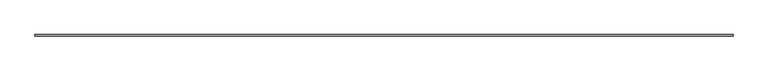
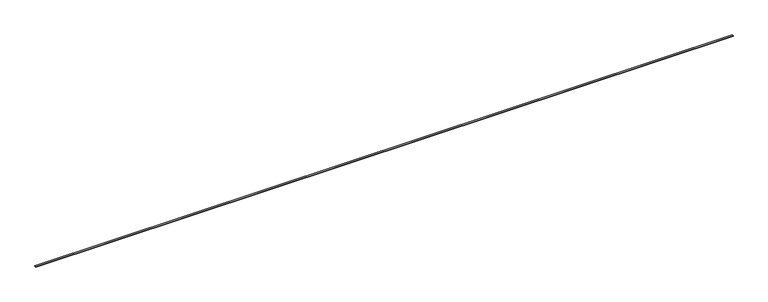
"""IFC4 building model written with IfcOpenShell, lengths in millimetres: proxy geometry, Generic Models 7:Generic Models 1:2:Generic Models 1:2 : Generic Models 7:Generic Models 1:337419:30 : Generic Models 7:Generic Models 1:2:Generic Models 1:2 : Generic Models 7:Generic Models 1:337419:306751."""

from ifc_helpers import new_model, si_unit, frame, origin, place, context, project, spatial, polyline, outline, extrude, source, transform, mapped, element, save


def generic_models_5c83f87b(model_context):
    return source(origin(), model_context, "Body", "SweptSolid", [
        extrude(outline(polyline([(0.0, -164.842211), (0.0, 0.0), (76200.0204281, 0.0), (76200.0204281, -164.842211), (0.0, -164.842211)])), frame((667506.057152, -567792.8921054, 8540.4597449), z_axis=(0.0, -0.041630544767773385, 0.9991330730900356), x_axis=(-1.0, 0.0, 0.0)), (0.0, 0.0, 1.0), 38.1),
    ])


if __name__ == "__main__":
    model = new_model("IFC4")
    model_context = context("Model", 3, world=origin())
    ifc_project = project(units=[si_unit("LENGTHUNIT", "METRE", prefix="MILLI")], contexts=[model_context])
    site = spatial("IfcSite", under=ifc_project)
    building = spatial("IfcBuilding", under=site)
    placement = place(None, origin())
    generic_models_shape = generic_models_5c83f87b(model_context)
    element("IfcBuildingElementProxy", 1, Name="Generic Models 7:Generic Models 1:2:Generic Models 1:2 : Generic Models 7:Generic Models 1:337419:30 : Generic Models 7:Generic Models 1:2:Generic Models 1:2 : Generic Models 7:Generic Models 1:337419:306751", ObjectType="Generic Models 7:Generic Models 1:2:Generic Models 1:2 : Generic Models 7:Generic Models 1:337419:30 : Generic Models 7:Generic Models 1:2:Generic Models 1:2 : Generic Models 7:Generic Models 1:337419:306751", at=placement, inside=building, context=model_context, shape_type="MappedRepresentation", body=[
        mapped(generic_models_shape, transform((0.0, 0.0, 0.0), x_axis=(1.0, 0.0, 0.0), y_axis=(0.0, 1.0, 0.0), z_axis=(0.0, 0.0, 1.0))),
    ])
    save(model, "model.ifc")

# Revit data of these elements
# Type "Generic Models 7:Generic Models 1:2:Generic Models 1:2 : Generic Models 7:Generic Models 1:337419:30 : Generic Models 7:Generic Models 1:2:Generic Models 1:2 : Generic Models 7:Generic Models 1:337419:306751"
#   NameOverride = "Generic Models 7:Generic Models 1:2:Generic Models 1:2 : Generic Models 7:Generic Models 1:337419:306751"
#   ObjectTypeOverride = "Generic Models 1:2 : Generic Models 7:Generic Models 1:337419"
#   Reference = "Generic Models 1"
#   Tag = "306751"
# Element 1 (IfcBuildingElementProxy, "Generic Models 7:Generic Models 1:2:Generic Models 1:2 : Generic Models 7:Generic Models 1:337419:30 : Generic Models 7:Generic Models 1:2:Generic Models 1:2 : Generic Models 7:Generic Models 1:337419:306751")
#   Materials on its faces: "FIRE RETARDTANT WOOD BLOCKING - SIZE AS NEC."
# Materials
#   "FIRE RETARDTANT WOOD BLOCKING - SIZE AS NEC.": class "Wood", colour RGB 144 113 62, transparency 0, Description = "Pinus Echinata", Cost = 0
